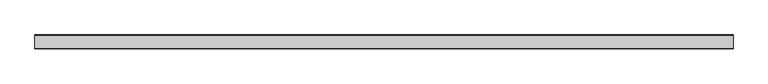
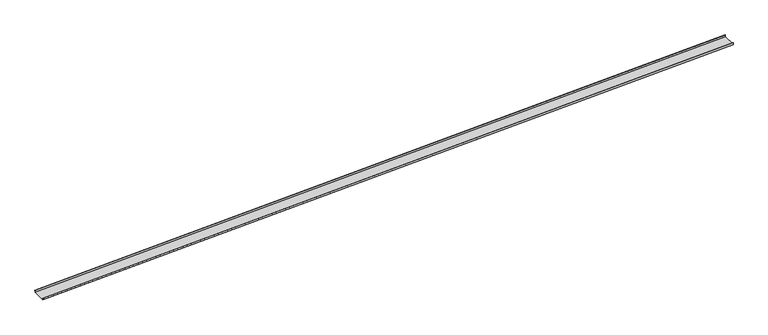
"""IFC4 building model written with IfcOpenShell, lengths in millimetres: proxy geometry, Generic Models 2:Generic Models 2:310765:Generic Models 2:310765 : Generic Models 2:Generic Models 2:310765:146 : Generic Models 2:Generic Models 2:310765:Generic Models 2:310765 : Generic Models 2:Generic Models 2:310765:300385."""

import ifcopenshell
import ifcopenshell.guid

model = None  # the IFC model being written
_history = None  # IfcOwnerHistory: only IFC2X3 demands one
_inside = {}  # id of a spatial element -> (the spatial element, [elements in it])
_under = {}  # id of a project, library or spatial element -> (it, [spatial elements below it])
_declared = {}  # id of a project -> (the project, [libraries it declares])
_typed = {}  # id of a type object -> (the type object, [elements of that type])
_made_of = {}  # id of a material, layer set ... -> (it, [elements and type objects made of it])


def new_model(schema):
    """Start an empty IFC model of exactly this schema.

    Asked for "IFC4X3", IfcOpenShell would pick the latest addendum, in which some entities
    have other attributes; the version numbers below select the first issue.
    IFC2X3 requires an IfcOwnerHistory on every rooted entity: one is made here for all.
    """
    global model, _history
    if schema == "IFC4X3":
        model = ifcopenshell.file(schema_version=(4, 3, 0, 0))
    else:
        model = ifcopenshell.file(schema=schema)
    _inside.clear()
    _under.clear()
    _declared.clear()
    _typed.clear()
    _made_of.clear()
    _history = None
    if model.schema == "IFC2X3":
        org = make("IfcOrganization", Name="unknown")
        user = make(
            "IfcPersonAndOrganization",
            ThePerson=make("IfcPerson", FamilyName="unknown"),
            TheOrganization=org,
        )
        app = make(
            "IfcApplication",
            ApplicationDeveloper=org,
            Version="unknown",
            ApplicationFullName="unknown",
            ApplicationIdentifier="unknown",
        )
        _history = make(
            "IfcOwnerHistory",
            OwningUser=user,
            OwningApplication=app,
            ChangeAction="ADDED",
            CreationDate=0,
        )
    return model


def make(cls, **values):
    """One entity of the class cls with the attributes given. An attribute that is None is left unset."""
    return model.create_entity(
        cls, **{name: value for name, value in values.items() if value is not None}
    )


def rooted(cls, **values):
    """An entity with a GlobalId (a new one), such as an element, a storey or a relation."""
    return make(cls, GlobalId=ifcopenshell.guid.new(), OwnerHistory=_history, **values)


def si_unit(unit_type, name, prefix=None):
    """IfcSIUnit, for example si_unit("LENGTHUNIT", "METRE", prefix="MILLI")."""
    return make("IfcSIUnit", UnitType=unit_type, Prefix=prefix, Name=name)


def assignment(units):
    """IfcUnitAssignment: the units of a project."""
    return None if units is None else make("IfcUnitAssignment", Units=units)


def point(xyz):
    """IfcCartesianPoint."""
    return None if xyz is None else make("IfcCartesianPoint", Coordinates=xyz)


def direction(xyz):
    """IfcDirection."""
    return None if xyz is None else make("IfcDirection", DirectionRatios=xyz)


def frame(location, z_axis=None, x_axis=None):
    """IfcAxis2Placement3D, a coordinate frame: its origin and axes. An axis left out is left unset."""
    return make(
        "IfcAxis2Placement3D",
        Location=point(location),
        Axis=direction(z_axis),
        RefDirection=direction(x_axis),
    )


def origin():
    """The frame at (0, 0, 0) with its axes left unset."""
    return frame((0.0, 0.0, 0.0))


def place(relative_to, where):
    """IfcLocalPlacement: puts the frame where relative to a parent placement (None: the world)."""
    return make(
        "IfcLocalPlacement", PlacementRelTo=relative_to, RelativePlacement=where
    )


def context(
    kind, dimensions, precision=None, world=None, true_north=None, identifier=None
):
    """IfcGeometricRepresentationContext, for example the 3D "Model" context."""
    return make(
        "IfcGeometricRepresentationContext",
        ContextIdentifier=identifier,
        ContextType=kind,
        CoordinateSpaceDimension=dimensions,
        Precision=precision,
        WorldCoordinateSystem=world,
        TrueNorth=true_north,
    )


def project(units=None, contexts=None):
    """IfcProject with its units and contexts."""
    return rooted(
        "IfcProject",
        Name="project",
        RepresentationContexts=contexts,
        UnitsInContext=assignment(units),
    )


def spatial(cls, under=None, at=None, **own):
    """A site, building, storey or space (cls), placed at a placement, below another one or the project."""
    s = rooted(cls, ObjectPlacement=at, **own)
    if under is not None:
        _under.setdefault(under.id(), (under, []))[1].append(s)
    return s


def polyline(points):
    """IfcPolyline through the points."""
    return make("IfcPolyline", Points=[point(p) for p in points])


def outline(outer, holes=None, kind="AREA"):
    """IfcArbitraryClosedProfileDef: a profile drawn as a closed curve; with holes, ...WithVoids."""
    if holes is None:
        return make("IfcArbitraryClosedProfileDef", ProfileType=kind, OuterCurve=outer)
    return make(
        "IfcArbitraryProfileDefWithVoids",
        ProfileType=kind,
        OuterCurve=outer,
        InnerCurves=holes,
    )


def extrude(swept, where, along, depth):
    """IfcExtrudedAreaSolid: the profile swept, set in the frame where, extruded along a direction by depth."""
    return make(
        "IfcExtrudedAreaSolid",
        SweptArea=swept,
        Position=where,
        ExtrudedDirection=direction(along),
        Depth=depth,
    )


def shape(context_of_items, identifier, shape_type, items):
    """IfcShapeRepresentation: the items that make up one representation, for example the "Body"."""
    return make(
        "IfcShapeRepresentation",
        ContextOfItems=context_of_items,
        RepresentationIdentifier=identifier,
        RepresentationType=shape_type,
        Items=items,
    )


def source(mapping_origin, context_of_items, identifier, shape_type, items):
    """IfcRepresentationMap: a shape defined once, which mapped items show again and again."""
    return make(
        "IfcRepresentationMap",
        MappingOrigin=mapping_origin,
        MappedRepresentation=shape(context_of_items, identifier, shape_type, items),
    )


def transform(
    local_origin,
    x_axis=None,
    y_axis=None,
    z_axis=None,
    scale=None,
    scale2=None,
    scale3=None,
    uniform=True,
):
    """IfcCartesianTransformationOperator3D, or its non-uniform kind. x_axis, y_axis, z_axis: its Axis1, 2, 3."""
    if uniform:
        return make(
            "IfcCartesianTransformationOperator3D",
            Axis1=direction(x_axis),
            Axis2=direction(y_axis),
            LocalOrigin=point(local_origin),
            Scale=scale,
            Axis3=direction(z_axis),
        )
    return make(
        "IfcCartesianTransformationOperator3DnonUniform",
        Axis1=direction(x_axis),
        Axis2=direction(y_axis),
        LocalOrigin=point(local_origin),
        Scale=scale,
        Axis3=direction(z_axis),
        Scale2=scale2,
        Scale3=scale3,
    )


def mapped(mapping_source, mapping_target):
    """IfcMappedItem: shows the shape of a source again, moved by a transform."""
    return make(
        "IfcMappedItem", MappingSource=mapping_source, MappingTarget=mapping_target
    )


def made_of(thing, what):
    """Note that an element or type object is made of a material, layer set ...; save() writes the relation."""
    if what is not None:
        _made_of.setdefault(what.id(), (what, []))[1].append(thing)
    return thing


def element(
    cls,
    number,
    at=None,
    inside=None,
    cuts=None,
    type_object=None,
    material=None,
    context=None,
    identifier="Body",
    shape_type=None,
    held_by="IfcProductDefinitionShape",
    body=None,
    shapes=None,
    **own,
):
    """One element of the class cls, such as IfcWall. Its Tag is "e" and its number.

    at: its placement. inside: the storey or other place that contains it. cuts: it is an
    opening in that element (IfcRelVoidsElement). A single representation is given by context,
    identifier, shape_type and body (its items); several are given by shapes. held_by: the class
    of the entity that holds the representations. save() writes the other relations.
    """
    e = rooted(cls, Tag="e%d" % number, ObjectPlacement=at, **own)
    if body is not None:
        shapes = [shape(context, identifier, shape_type, body)]
    if shapes is not None:
        e.Representation = make(held_by, Representations=shapes)
    if inside is not None:
        _inside.setdefault(inside.id(), (inside, []))[1].append(e)
    if cuts is not None:
        rooted(
            "IfcRelVoidsElement", RelatingBuildingElement=cuts, RelatedOpeningElement=e
        )
    if type_object is not None:
        _typed.setdefault(type_object.id(), (type_object, []))[1].append(e)
    return made_of(e, material)


def aggregate(whole, parts):
    """IfcRelAggregates: a whole, such as a stair, and the parts it consists of."""
    return rooted("IfcRelAggregates", RelatingObject=whole, RelatedObjects=parts)


def save(model, path):
    """Write the relations noted so far, then the file.

    IfcRelAggregates (storeys below a building ...), IfcRelContainedInSpatialStructure (elements
    in a storey), IfcRelDefinesByType, IfcRelAssociatesMaterial and IfcRelDeclares: one each for
    every whole, place, type object, material and project.
    """
    for whole, parts in _under.values():
        aggregate(whole, parts)
    for where, things in _inside.values():
        rooted(
            "IfcRelContainedInSpatialStructure",
            RelatedElements=things,
            RelatingStructure=where,
        )
    for kind, things in _typed.values():
        rooted("IfcRelDefinesByType", RelatedObjects=things, RelatingType=kind)
    for what, things in _made_of.values():
        rooted("IfcRelAssociatesMaterial", RelatedObjects=things, RelatingMaterial=what)
    for by, libraries in _declared.values():
        rooted("IfcRelDeclares", RelatingContext=by, RelatedDefinitions=libraries)
    model.write(path)


def generic_models_b84086ad(model_context):
    return source(origin(), model_context, "Body", "SweptSolid", [
        extrude(outline(polyline([(1.5875, 0.0), (1.5875, 50.8), (407.9875, 50.8), (407.9875, 1.5874999), (396.875, 1.5874999), (396.875, 11.1125), (398.4625, 11.1125), (398.4625, 3.175), (406.4, 3.175), (406.4, 49.2124999), (3.175, 49.2124999), (3.175, -1.5875), (-14.2875, -1.5875), (-14.2875, 9.525), (-12.7, 9.525), (-12.7, 0.0), (1.5875, 0.0)])), frame((558060.6329583, -578114.072634, 3904.6995643), z_axis=(0.9991330730923568, 0.0, 0.041630544712067834), x_axis=(0.0, -1.0, 0.0)), (0.0, 0.0, 1.0), 21007.9629603),
    ])


if __name__ == "__main__":
    model = new_model("IFC4")
    model_context = context("Model", 3, world=origin())
    ifc_project = project(units=[si_unit("LENGTHUNIT", "METRE", prefix="MILLI")], contexts=[model_context])
    site = spatial("IfcSite", under=ifc_project)
    building = spatial("IfcBuilding", under=site)
    placement = place(None, origin())
    generic_models_shape = generic_models_b84086ad(model_context)
    element("IfcBuildingElementProxy", 1, Name="Generic Models 2:Generic Models 2:310765:Generic Models 2:310765 : Generic Models 2:Generic Models 2:310765:146 : Generic Models 2:Generic Models 2:310765:Generic Models 2:310765 : Generic Models 2:Generic Models 2:310765:300385", ObjectType="Generic Models 2:Generic Models 2:310765:Generic Models 2:310765 : Generic Models 2:Generic Models 2:310765:146 : Generic Models 2:Generic Models 2:310765:Generic Models 2:310765 : Generic Models 2:Generic Models 2:310765:300385", at=placement, inside=building, context=model_context, shape_type="MappedRepresentation", body=[
        mapped(generic_models_shape, transform((0.0, 0.0, 0.0), x_axis=(1.0, 0.0, 0.0), y_axis=(0.0, 1.0, 0.0), z_axis=(0.0, 0.0, 1.0))),
    ])
    save(model, "model.ifc")

# Revit data of these elements
# Type "Generic Models 2:Generic Models 2:310765:Generic Models 2:310765 : Generic Models 2:Generic Models 2:310765:146 : Generic Models 2:Generic Models 2:310765:Generic Models 2:310765 : Generic Models 2:Generic Models 2:310765:300385"
#   NameOverride = "Generic Models 2:Generic Models 2:310765:Generic Models 2:310765 : Generic Models 2:Generic Models 2:310765:300385"
#   ObjectTypeOverride = "Generic Models 2:310765 : Generic Models 2:Generic Models 2:310765"
#   Reference = "Generic Models 2"
#   Tag = "300385"
# Element 1 (IfcBuildingElementProxy, "Generic Models 2:Generic Models 2:310765:Generic Models 2:310765 : Generic Models 2:Generic Models 2:310765:146 : Generic Models 2:Generic Models 2:310765:Generic Models 2:310765 : Generic Models 2:Generic Models 2:310765:300385")
#   Materials on its faces: "STRUCTURAL STANDING SEAM SHEET METAL ROOFING - BATTENLOK - COLOR T.B.D."
# Materials
#   "STRUCTURAL STANDING SEAM SHEET METAL ROOFING - BATTENLOK - COLOR T.B.D.": class "Generic", colour RGB 120 120 120, transparency 0, Cost = 0
